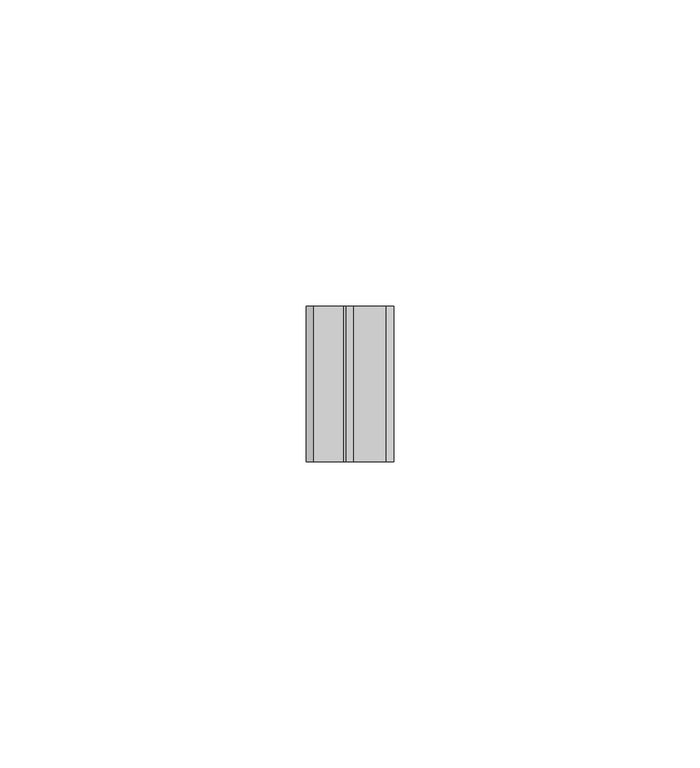
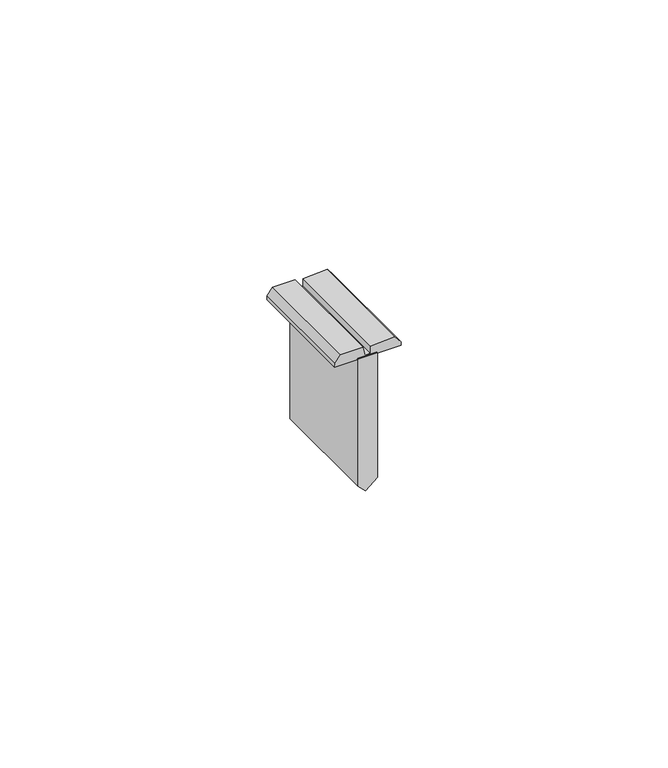
"""IFC4 building model written with IfcOpenShell, lengths in millimetres: proxy geometry, FASTENER006 5976 : FASTENER006 5976."""

from ifc_helpers import new_model, si_unit, frame, origin, place, context, project, spatial, polyline, outline, extrude, source, transform, mapped, element, save


def generic_models_f031ca55(model_context):
    return source(origin(), model_context, "Body", "SweptSolid", [
        extrude(outline(polyline([(42577.1576024, 5870.6890035), (42548.1988623, 5870.6890035), (42546.5833096, 5872.3460181), (42548.7638676, 5874.895922), (42577.1576024, 5874.895922), (42577.1576024, 5870.6890035)])), frame((0.0, -1078.2906574, 0.0), z_axis=(0.0, 1.0, 0.0), x_axis=(0.0, 0.0, 1.0)), (0.0, 0.0, 1.0), 25.4),
        extrude(outline(polyline([(42577.1576024, 5879.9417891), (42577.9674245, 5879.9417891), (42579.5612959, 5878.7030871), (42579.1650604, 5873.4174049), (42577.5756297, 5873.4174049), (42577.5756297, 5872.1703), (42579.587761, 5871.7740645), (42579.587761, 5866.8949826), (42577.9938896, 5865.6562805), (42577.1576024, 5865.6454839), (42577.1576024, 5879.9417891)])), frame((0.0, -1078.2906574, 0.0), z_axis=(0.0, 1.0, 0.0), x_axis=(0.0, 0.0, 1.0)), (0.0, 0.0, 1.0), 25.4),
    ])


if __name__ == "__main__":
    model = new_model("IFC4")
    model_context = context("Model", 3, world=origin())
    ifc_project = project(units=[si_unit("LENGTHUNIT", "METRE", prefix="MILLI")], contexts=[model_context])
    site = spatial("IfcSite", under=ifc_project)
    building = spatial("IfcBuilding", under=site)
    placement = place(None, origin())
    generic_models_shape = generic_models_f031ca55(model_context)
    element("IfcBuildingElementProxy", 1, Name="FASTENER006 5976 : FASTENER006 5976", ObjectType="FASTENER006 5976 : FASTENER006 5976", at=placement, inside=building, context=model_context, shape_type="MappedRepresentation", body=[
        mapped(generic_models_shape, transform((0.0, 0.0, 0.0), x_axis=(1.0, 0.0, 0.0), y_axis=(0.0, 1.0, 0.0), z_axis=(0.0, 0.0, 1.0))),
    ])
    save(model, "model.ifc")

# Revit data of these elements
# Type "FASTENER006 5976 : FASTENER006 5976"
#   NameOverride = "FASTENER006"
# Element 1 (IfcBuildingElementProxy, "FASTENER006 5976 : FASTENER006 5976")
#   Materials on its faces: "ENGINEERED PANCAKE HEAD FASTENER (NOT BY AEP-SPAN) @ 12\" O.C."
# Materials
#   "ENGINEERED PANCAKE HEAD FASTENER (NOT BY AEP-SPAN) @ 12\" O.C.": class "Unassigned", colour RGB 255 255 255, transparency 0
